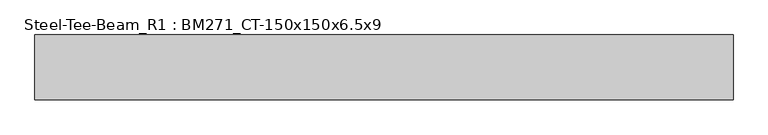
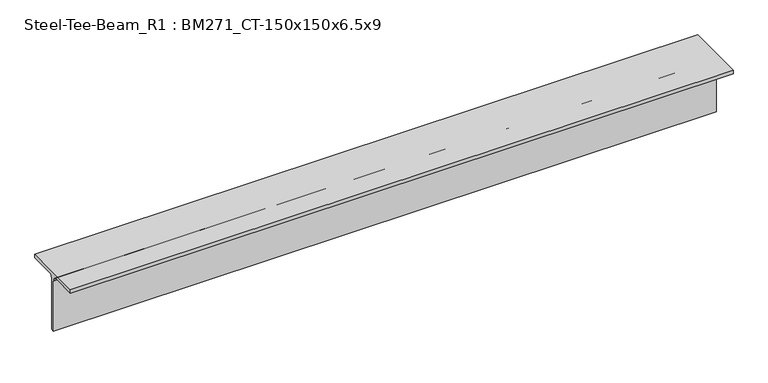
"""IFC4 building model written with IfcOpenShell, lengths in millimetres: member geometry, Steel-Tee-Beam_R1 : BM271_CT-150x150x6.5x9."""

from ifc_helpers import new_model, si_unit, point, frame, frame_2d, origin, place, context, project, spatial, polyline, circle_curve, trimmed, segment, composite_curve, outline, extrude, source, transform, mapped, element, save


def steel_tee_beam_r1_bm271_ct_150x150x6_5x9_4170945b(model_context):
    return source(origin(), model_context, "Body", "SweptSolid", [
        extrude(outline(composite_curve([segment(polyline([(75.0, 75.0), (75.0, 66.0), (16.25, 66.0)]), True, "CONTINUOUS"), segment(trimmed(circle_curve(frame_2d((16.25, 53.0)), 13.0), [point((16.25, 66.0))], [point((3.25, 53.0))], True, "CARTESIAN"), True, "CONTINUOUS"), segment(polyline([(3.25, 53.0), (3.25, -75.0), (-3.25, -75.0), (-3.25, 53.0)]), True, "CONTINUOUS"), segment(trimmed(circle_curve(frame_2d((-16.25, 53.0)), 13.0), [point((-3.25, 53.0))], [point((-16.25, 66.0))], True, "CARTESIAN"), True, "CONTINUOUS"), segment(polyline([(-16.25, 66.0), (-75.0, 66.0), (-75.0, 75.0), (75.0, 75.0)]), True, "CONTINUOUS")], self_intersect=False)), frame((-807.1037633, 0.0, 0.0), z_axis=(1.0, 0.0, 0.0), x_axis=(0.0, 1.0, 0.0)), (0.0, 0.0, 1.0), 1614.2075266),
    ])


if __name__ == "__main__":
    model = new_model("IFC4")
    model_context = context("Model", 3, world=origin())
    ifc_project = project(units=[si_unit("LENGTHUNIT", "METRE", prefix="MILLI")], contexts=[model_context])
    site = spatial("IfcSite", under=ifc_project)
    building = spatial("IfcBuilding", under=site)
    placement = place(None, origin())
    steel_tee_beam_r1_bm271_ct_150x150x6_5x9_shape = steel_tee_beam_r1_bm271_ct_150x150x6_5x9_4170945b(model_context)
    element("IfcMember", 1, ObjectType="Steel-Tee-Beam_R1 : BM271_CT-150x150x6.5x9", at=placement, inside=building, context=model_context, shape_type="MappedRepresentation", body=[
        mapped(steel_tee_beam_r1_bm271_ct_150x150x6_5x9_shape, transform((0.0, 0.0, 0.0), x_axis=(1.0, 0.0, 0.0), y_axis=(0.0, 1.0, 0.0), z_axis=(0.0, 0.0, 1.0))),
    ])
    save(model, "model.ifc")

# Revit data of these elements
# Type "Steel-Tee-Beam_R1 : BM271_CT-150x150x6.5x9"
#   Keynote = "CT-150x150x6.5x9"
#   Surface Area = 0.588841 m²/m
#   Section Area = 23.3904 cm²
#   Mass per Unit Length = 18.3614 kg/m
#   Length [instance default] = 1.5240 m
#   bf = 0.1500 m
#   d = 0.1500 m
#   k = 0.0220 m
#   r = 0.0130 m
#   tf = 0.0090 m
#   tw = 0.0065 m
#   hec_material4 [instance default] = none
#   hec_material3 [instance default] = none
#   hec_material2 [instance default] = none
#   hec_material1 [instance default] = none
#   Structural Material [instance default] = Steel, 45-345
#   Assembly Code = ""
# Element 1 (IfcMember, "Steel-Tee-Beam_R1 : BM271_CT-150x150x6.5x9")
#   Structural Material = none
# Materials
#   "Steel, 45-345": class "Metal", colour RGB 189 187 185, transparency 0, Description = "Steel 345 MPa", Cost = 0
